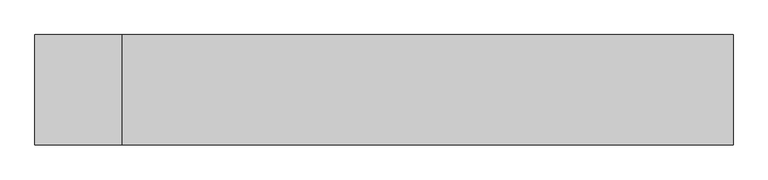
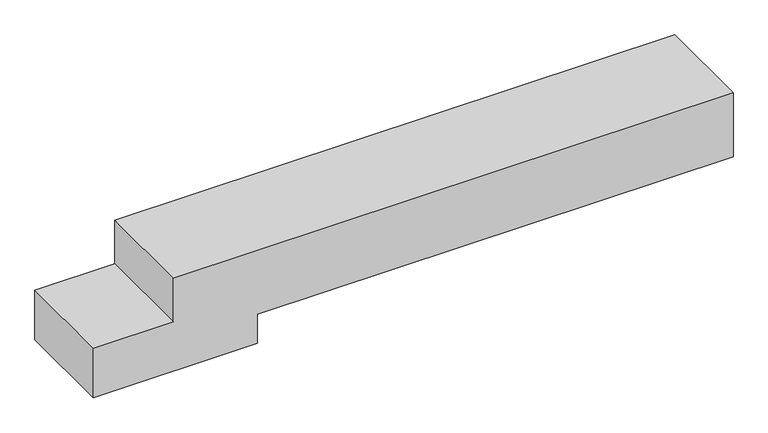
"""IFC4 building model written with IfcOpenShell, lengths in millimetres: proxy geometry, Generic Models 243:Generic Models 243:154672 : Generic Models 243:Generic Models 243:154672."""

import ifcopenshell
import ifcopenshell.guid

model = None  # the IFC model being written
_history = None  # IfcOwnerHistory: only IFC2X3 demands one
_inside = {}  # id of a spatial element -> (the spatial element, [elements in it])
_under = {}  # id of a project, library or spatial element -> (it, [spatial elements below it])
_declared = {}  # id of a project -> (the project, [libraries it declares])
_typed = {}  # id of a type object -> (the type object, [elements of that type])
_made_of = {}  # id of a material, layer set ... -> (it, [elements and type objects made of it])


def new_model(schema):
    """Start an empty IFC model of exactly this schema.

    Asked for "IFC4X3", IfcOpenShell would pick the latest addendum, in which some entities
    have other attributes; the version numbers below select the first issue.
    IFC2X3 requires an IfcOwnerHistory on every rooted entity: one is made here for all.
    """
    global model, _history
    if schema == "IFC4X3":
        model = ifcopenshell.file(schema_version=(4, 3, 0, 0))
    else:
        model = ifcopenshell.file(schema=schema)
    _inside.clear()
    _under.clear()
    _declared.clear()
    _typed.clear()
    _made_of.clear()
    _history = None
    if model.schema == "IFC2X3":
        org = make("IfcOrganization", Name="unknown")
        user = make(
            "IfcPersonAndOrganization",
            ThePerson=make("IfcPerson", FamilyName="unknown"),
            TheOrganization=org,
        )
        app = make(
            "IfcApplication",
            ApplicationDeveloper=org,
            Version="unknown",
            ApplicationFullName="unknown",
            ApplicationIdentifier="unknown",
        )
        _history = make(
            "IfcOwnerHistory",
            OwningUser=user,
            OwningApplication=app,
            ChangeAction="ADDED",
            CreationDate=0,
        )
    return model


def make(cls, **values):
    """One entity of the class cls with the attributes given. An attribute that is None is left unset."""
    return model.create_entity(
        cls, **{name: value for name, value in values.items() if value is not None}
    )


def rooted(cls, **values):
    """An entity with a GlobalId (a new one), such as an element, a storey or a relation."""
    return make(cls, GlobalId=ifcopenshell.guid.new(), OwnerHistory=_history, **values)


def si_unit(unit_type, name, prefix=None):
    """IfcSIUnit, for example si_unit("LENGTHUNIT", "METRE", prefix="MILLI")."""
    return make("IfcSIUnit", UnitType=unit_type, Prefix=prefix, Name=name)


def assignment(units):
    """IfcUnitAssignment: the units of a project."""
    return None if units is None else make("IfcUnitAssignment", Units=units)


def point(xyz):
    """IfcCartesianPoint."""
    return None if xyz is None else make("IfcCartesianPoint", Coordinates=xyz)


def direction(xyz):
    """IfcDirection."""
    return None if xyz is None else make("IfcDirection", DirectionRatios=xyz)


def frame(location, z_axis=None, x_axis=None):
    """IfcAxis2Placement3D, a coordinate frame: its origin and axes. An axis left out is left unset."""
    return make(
        "IfcAxis2Placement3D",
        Location=point(location),
        Axis=direction(z_axis),
        RefDirection=direction(x_axis),
    )


def origin():
    """The frame at (0, 0, 0) with its axes left unset."""
    return frame((0.0, 0.0, 0.0))


def place(relative_to, where):
    """IfcLocalPlacement: puts the frame where relative to a parent placement (None: the world)."""
    return make(
        "IfcLocalPlacement", PlacementRelTo=relative_to, RelativePlacement=where
    )


def context(
    kind, dimensions, precision=None, world=None, true_north=None, identifier=None
):
    """IfcGeometricRepresentationContext, for example the 3D "Model" context."""
    return make(
        "IfcGeometricRepresentationContext",
        ContextIdentifier=identifier,
        ContextType=kind,
        CoordinateSpaceDimension=dimensions,
        Precision=precision,
        WorldCoordinateSystem=world,
        TrueNorth=true_north,
    )


def project(units=None, contexts=None):
    """IfcProject with its units and contexts."""
    return rooted(
        "IfcProject",
        Name="project",
        RepresentationContexts=contexts,
        UnitsInContext=assignment(units),
    )


def spatial(cls, under=None, at=None, **own):
    """A site, building, storey or space (cls), placed at a placement, below another one or the project."""
    s = rooted(cls, ObjectPlacement=at, **own)
    if under is not None:
        _under.setdefault(under.id(), (under, []))[1].append(s)
    return s


def polyline(points):
    """IfcPolyline through the points."""
    return make("IfcPolyline", Points=[point(p) for p in points])


def outline(outer, holes=None, kind="AREA"):
    """IfcArbitraryClosedProfileDef: a profile drawn as a closed curve; with holes, ...WithVoids."""
    if holes is None:
        return make("IfcArbitraryClosedProfileDef", ProfileType=kind, OuterCurve=outer)
    return make(
        "IfcArbitraryProfileDefWithVoids",
        ProfileType=kind,
        OuterCurve=outer,
        InnerCurves=holes,
    )


def extrude(swept, where, along, depth):
    """IfcExtrudedAreaSolid: the profile swept, set in the frame where, extruded along a direction by depth."""
    return make(
        "IfcExtrudedAreaSolid",
        SweptArea=swept,
        Position=where,
        ExtrudedDirection=direction(along),
        Depth=depth,
    )


def shape(context_of_items, identifier, shape_type, items):
    """IfcShapeRepresentation: the items that make up one representation, for example the "Body"."""
    return make(
        "IfcShapeRepresentation",
        ContextOfItems=context_of_items,
        RepresentationIdentifier=identifier,
        RepresentationType=shape_type,
        Items=items,
    )


def source(mapping_origin, context_of_items, identifier, shape_type, items):
    """IfcRepresentationMap: a shape defined once, which mapped items show again and again."""
    return make(
        "IfcRepresentationMap",
        MappingOrigin=mapping_origin,
        MappedRepresentation=shape(context_of_items, identifier, shape_type, items),
    )


def transform(
    local_origin,
    x_axis=None,
    y_axis=None,
    z_axis=None,
    scale=None,
    scale2=None,
    scale3=None,
    uniform=True,
):
    """IfcCartesianTransformationOperator3D, or its non-uniform kind. x_axis, y_axis, z_axis: its Axis1, 2, 3."""
    if uniform:
        return make(
            "IfcCartesianTransformationOperator3D",
            Axis1=direction(x_axis),
            Axis2=direction(y_axis),
            LocalOrigin=point(local_origin),
            Scale=scale,
            Axis3=direction(z_axis),
        )
    return make(
        "IfcCartesianTransformationOperator3DnonUniform",
        Axis1=direction(x_axis),
        Axis2=direction(y_axis),
        LocalOrigin=point(local_origin),
        Scale=scale,
        Axis3=direction(z_axis),
        Scale2=scale2,
        Scale3=scale3,
    )


def mapped(mapping_source, mapping_target):
    """IfcMappedItem: shows the shape of a source again, moved by a transform."""
    return make(
        "IfcMappedItem", MappingSource=mapping_source, MappingTarget=mapping_target
    )


def made_of(thing, what):
    """Note that an element or type object is made of a material, layer set ...; save() writes the relation."""
    if what is not None:
        _made_of.setdefault(what.id(), (what, []))[1].append(thing)
    return thing


def element(
    cls,
    number,
    at=None,
    inside=None,
    cuts=None,
    type_object=None,
    material=None,
    context=None,
    identifier="Body",
    shape_type=None,
    held_by="IfcProductDefinitionShape",
    body=None,
    shapes=None,
    **own,
):
    """One element of the class cls, such as IfcWall. Its Tag is "e" and its number.

    at: its placement. inside: the storey or other place that contains it. cuts: it is an
    opening in that element (IfcRelVoidsElement). A single representation is given by context,
    identifier, shape_type and body (its items); several are given by shapes. held_by: the class
    of the entity that holds the representations. save() writes the other relations.
    """
    e = rooted(cls, Tag="e%d" % number, ObjectPlacement=at, **own)
    if body is not None:
        shapes = [shape(context, identifier, shape_type, body)]
    if shapes is not None:
        e.Representation = make(held_by, Representations=shapes)
    if inside is not None:
        _inside.setdefault(inside.id(), (inside, []))[1].append(e)
    if cuts is not None:
        rooted(
            "IfcRelVoidsElement", RelatingBuildingElement=cuts, RelatedOpeningElement=e
        )
    if type_object is not None:
        _typed.setdefault(type_object.id(), (type_object, []))[1].append(e)
    return made_of(e, material)


def aggregate(whole, parts):
    """IfcRelAggregates: a whole, such as a stair, and the parts it consists of."""
    return rooted("IfcRelAggregates", RelatingObject=whole, RelatedObjects=parts)


def save(model, path):
    """Write the relations noted so far, then the file.

    IfcRelAggregates (storeys below a building ...), IfcRelContainedInSpatialStructure (elements
    in a storey), IfcRelDefinesByType, IfcRelAssociatesMaterial and IfcRelDeclares: one each for
    every whole, place, type object, material and project.
    """
    for whole, parts in _under.values():
        aggregate(whole, parts)
    for where, things in _inside.values():
        rooted(
            "IfcRelContainedInSpatialStructure",
            RelatedElements=things,
            RelatingStructure=where,
        )
    for kind, things in _typed.values():
        rooted("IfcRelDefinesByType", RelatedObjects=things, RelatingType=kind)
    for what, things in _made_of.values():
        rooted("IfcRelAssociatesMaterial", RelatedObjects=things, RelatingMaterial=what)
    for by, libraries in _declared.values():
        rooted("IfcRelDeclares", RelatingContext=by, RelatedDefinitions=libraries)
    model.write(path)


def generic_models_7add1f84(model_context):
    return source(origin(), model_context, "Body", "SweptSolid", [
        extrude(outline(polyline([(138.1125, 1584.203213), (138.1125, -104.896787), (0.0, -104.896787), (0.0, -346.196787), (-158.75, -346.196787), (-158.75, 149.103213), (-65.0875, 149.103213), (-65.0875, 1584.203213), (138.1125, 1584.203213)])), frame((0.0, 4450.212823, 0.0), z_axis=(0.0, 1.0, 0.0), x_axis=(0.0, 0.0, 1.0)), (0.0, 0.0, 1.0), 304.8),
    ])


if __name__ == "__main__":
    model = new_model("IFC4")
    model_context = context("Model", 3, world=origin())
    ifc_project = project(units=[si_unit("LENGTHUNIT", "METRE", prefix="MILLI")], contexts=[model_context])
    site = spatial("IfcSite", under=ifc_project)
    building = spatial("IfcBuilding", under=site)
    placement = place(None, origin())
    generic_models_shape = generic_models_7add1f84(model_context)
    element("IfcBuildingElementProxy", 1, Name="Generic Models 243:Generic Models 243:154672 : Generic Models 243:Generic Models 243:154672", ObjectType="Generic Models 243:Generic Models 243:154672 : Generic Models 243:Generic Models 243:154672", at=placement, inside=building, context=model_context, shape_type="MappedRepresentation", body=[
        mapped(generic_models_shape, transform((0.0, 0.0, 0.0), x_axis=(1.0, 0.0, 0.0), y_axis=(0.0, 1.0, 0.0), z_axis=(0.0, 0.0, 1.0))),
    ])
    save(model, "model.ifc")

# Revit data of these elements
# Type "Generic Models 243:Generic Models 243:154672 : Generic Models 243:Generic Models 243:154672"
#   NameOverride = "Generic Models 243:Generic Models 243:154672"
#   ObjectTypeOverride = "Generic Models 243:Generic Models 243"
#   Reference = "Generic Models 243"
#   Category = "Generic Models"
#   Tag = "154672"
# Element 1 (IfcBuildingElementProxy, "Generic Models 243:Generic Models 243:154672 : Generic Models 243:Generic Models 243:154672")
#   Materials on its faces: "_ 8\" CONCRETE SLAB W/ GRADE BEAM (SEE STRUCT. DWGS) 10051"
# Materials
#   "_ 8\" CONCRETE SLAB W/ GRADE BEAM (SEE STRUCT. DWGS) 10051": class "Unassigned", colour RGB 191 191 191, transparency 0
